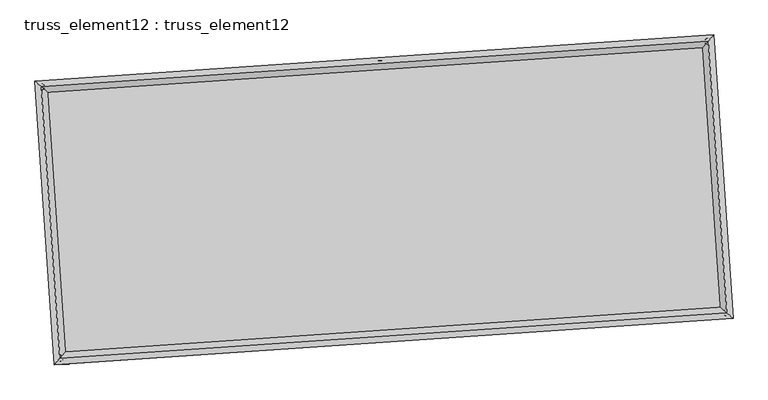
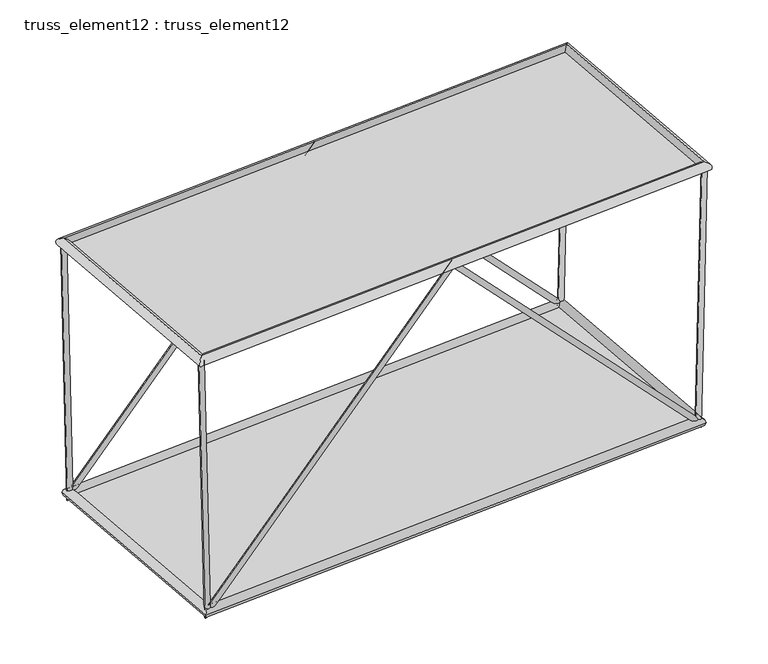
"""IFC4 building model written with IfcOpenShell, lengths in millimetres: plate geometry, truss_element12 : truss_element12."""

import ifcopenshell
import ifcopenshell.guid

model = None  # the IFC model being written
_history = None  # IfcOwnerHistory: only IFC2X3 demands one
_inside = {}  # id of a spatial element -> (the spatial element, [elements in it])
_under = {}  # id of a project, library or spatial element -> (it, [spatial elements below it])
_declared = {}  # id of a project -> (the project, [libraries it declares])
_typed = {}  # id of a type object -> (the type object, [elements of that type])
_made_of = {}  # id of a material, layer set ... -> (it, [elements and type objects made of it])


def new_model(schema):
    """Start an empty IFC model of exactly this schema.

    Asked for "IFC4X3", IfcOpenShell would pick the latest addendum, in which some entities
    have other attributes; the version numbers below select the first issue.
    IFC2X3 requires an IfcOwnerHistory on every rooted entity: one is made here for all.
    """
    global model, _history
    if schema == "IFC4X3":
        model = ifcopenshell.file(schema_version=(4, 3, 0, 0))
    else:
        model = ifcopenshell.file(schema=schema)
    _inside.clear()
    _under.clear()
    _declared.clear()
    _typed.clear()
    _made_of.clear()
    _history = None
    if model.schema == "IFC2X3":
        org = make("IfcOrganization", Name="unknown")
        user = make(
            "IfcPersonAndOrganization",
            ThePerson=make("IfcPerson", FamilyName="unknown"),
            TheOrganization=org,
        )
        app = make(
            "IfcApplication",
            ApplicationDeveloper=org,
            Version="unknown",
            ApplicationFullName="unknown",
            ApplicationIdentifier="unknown",
        )
        _history = make(
            "IfcOwnerHistory",
            OwningUser=user,
            OwningApplication=app,
            ChangeAction="ADDED",
            CreationDate=0,
        )
    return model


def make(cls, **values):
    """One entity of the class cls with the attributes given. An attribute that is None is left unset."""
    return model.create_entity(
        cls, **{name: value for name, value in values.items() if value is not None}
    )


def rooted(cls, **values):
    """An entity with a GlobalId (a new one), such as an element, a storey or a relation."""
    return make(cls, GlobalId=ifcopenshell.guid.new(), OwnerHistory=_history, **values)


def si_unit(unit_type, name, prefix=None):
    """IfcSIUnit, for example si_unit("LENGTHUNIT", "METRE", prefix="MILLI")."""
    return make("IfcSIUnit", UnitType=unit_type, Prefix=prefix, Name=name)


def assignment(units):
    """IfcUnitAssignment: the units of a project."""
    return None if units is None else make("IfcUnitAssignment", Units=units)


def point(xyz):
    """IfcCartesianPoint."""
    return None if xyz is None else make("IfcCartesianPoint", Coordinates=xyz)


def direction(xyz):
    """IfcDirection."""
    return None if xyz is None else make("IfcDirection", DirectionRatios=xyz)


def frame(location, z_axis=None, x_axis=None):
    """IfcAxis2Placement3D, a coordinate frame: its origin and axes. An axis left out is left unset."""
    return make(
        "IfcAxis2Placement3D",
        Location=point(location),
        Axis=direction(z_axis),
        RefDirection=direction(x_axis),
    )


def origin():
    """The frame at (0, 0, 0) with its axes left unset."""
    return frame((0.0, 0.0, 0.0))


def origin_with_axes():
    """The frame at (0, 0, 0) with the z axis (0, 0, 1) and the x axis (1, 0, 0) written out."""
    return frame((0.0, 0.0, 0.0), z_axis=(0.0, 0.0, 1.0), x_axis=(1.0, 0.0, 0.0))


def place(relative_to, where):
    """IfcLocalPlacement: puts the frame where relative to a parent placement (None: the world)."""
    return make(
        "IfcLocalPlacement", PlacementRelTo=relative_to, RelativePlacement=where
    )


def context(
    kind, dimensions, precision=None, world=None, true_north=None, identifier=None
):
    """IfcGeometricRepresentationContext, for example the 3D "Model" context."""
    return make(
        "IfcGeometricRepresentationContext",
        ContextIdentifier=identifier,
        ContextType=kind,
        CoordinateSpaceDimension=dimensions,
        Precision=precision,
        WorldCoordinateSystem=world,
        TrueNorth=true_north,
    )


def project(units=None, contexts=None):
    """IfcProject with its units and contexts."""
    return rooted(
        "IfcProject",
        Name="project",
        RepresentationContexts=contexts,
        UnitsInContext=assignment(units),
    )


def spatial(cls, under=None, at=None, **own):
    """A site, building, storey or space (cls), placed at a placement, below another one or the project."""
    s = rooted(cls, ObjectPlacement=at, **own)
    if under is not None:
        _under.setdefault(under.id(), (under, []))[1].append(s)
    return s


def polyline(points):
    """IfcPolyline through the points."""
    return make("IfcPolyline", Points=[point(p) for p in points])


def circle_curve(where, radius):
    """IfcCircle in the frame where."""
    return make("IfcCircle", Position=where, Radius=radius)


def ellipse_curve(where, semi_axis1, semi_axis2):
    """IfcEllipse in the frame where."""
    return make(
        "IfcEllipse", Position=where, SemiAxis1=semi_axis1, SemiAxis2=semi_axis2
    )


def outline(outer, holes=None, kind="AREA"):
    """IfcArbitraryClosedProfileDef: a profile drawn as a closed curve; with holes, ...WithVoids."""
    if holes is None:
        return make("IfcArbitraryClosedProfileDef", ProfileType=kind, OuterCurve=outer)
    return make(
        "IfcArbitraryProfileDefWithVoids",
        ProfileType=kind,
        OuterCurve=outer,
        InnerCurves=holes,
    )


def extrude(swept, where, along, depth):
    """IfcExtrudedAreaSolid: the profile swept, set in the frame where, extruded along a direction by depth."""
    return make(
        "IfcExtrudedAreaSolid",
        SweptArea=swept,
        Position=where,
        ExtrudedDirection=direction(along),
        Depth=depth,
    )


def shape(context_of_items, identifier, shape_type, items):
    """IfcShapeRepresentation: the items that make up one representation, for example the "Body"."""
    return make(
        "IfcShapeRepresentation",
        ContextOfItems=context_of_items,
        RepresentationIdentifier=identifier,
        RepresentationType=shape_type,
        Items=items,
    )


def source(mapping_origin, context_of_items, identifier, shape_type, items):
    """IfcRepresentationMap: a shape defined once, which mapped items show again and again."""
    return make(
        "IfcRepresentationMap",
        MappingOrigin=mapping_origin,
        MappedRepresentation=shape(context_of_items, identifier, shape_type, items),
    )


def transform(
    local_origin,
    x_axis=None,
    y_axis=None,
    z_axis=None,
    scale=None,
    scale2=None,
    scale3=None,
    uniform=True,
):
    """IfcCartesianTransformationOperator3D, or its non-uniform kind. x_axis, y_axis, z_axis: its Axis1, 2, 3."""
    if uniform:
        return make(
            "IfcCartesianTransformationOperator3D",
            Axis1=direction(x_axis),
            Axis2=direction(y_axis),
            LocalOrigin=point(local_origin),
            Scale=scale,
            Axis3=direction(z_axis),
        )
    return make(
        "IfcCartesianTransformationOperator3DnonUniform",
        Axis1=direction(x_axis),
        Axis2=direction(y_axis),
        LocalOrigin=point(local_origin),
        Scale=scale,
        Axis3=direction(z_axis),
        Scale2=scale2,
        Scale3=scale3,
    )


def mapped(mapping_source, mapping_target):
    """IfcMappedItem: shows the shape of a source again, moved by a transform."""
    return make(
        "IfcMappedItem", MappingSource=mapping_source, MappingTarget=mapping_target
    )


def made_of(thing, what):
    """Note that an element or type object is made of a material, layer set ...; save() writes the relation."""
    if what is not None:
        _made_of.setdefault(what.id(), (what, []))[1].append(thing)
    return thing


def element(
    cls,
    number,
    at=None,
    inside=None,
    cuts=None,
    type_object=None,
    material=None,
    context=None,
    identifier="Body",
    shape_type=None,
    held_by="IfcProductDefinitionShape",
    body=None,
    shapes=None,
    **own,
):
    """One element of the class cls, such as IfcWall. Its Tag is "e" and its number.

    at: its placement. inside: the storey or other place that contains it. cuts: it is an
    opening in that element (IfcRelVoidsElement). A single representation is given by context,
    identifier, shape_type and body (its items); several are given by shapes. held_by: the class
    of the entity that holds the representations. save() writes the other relations.
    """
    e = rooted(cls, Tag="e%d" % number, ObjectPlacement=at, **own)
    if body is not None:
        shapes = [shape(context, identifier, shape_type, body)]
    if shapes is not None:
        e.Representation = make(held_by, Representations=shapes)
    if inside is not None:
        _inside.setdefault(inside.id(), (inside, []))[1].append(e)
    if cuts is not None:
        rooted(
            "IfcRelVoidsElement", RelatingBuildingElement=cuts, RelatedOpeningElement=e
        )
    if type_object is not None:
        _typed.setdefault(type_object.id(), (type_object, []))[1].append(e)
    return made_of(e, material)


def aggregate(whole, parts):
    """IfcRelAggregates: a whole, such as a stair, and the parts it consists of."""
    return rooted("IfcRelAggregates", RelatingObject=whole, RelatedObjects=parts)


def save(model, path):
    """Write the relations noted so far, then the file.

    IfcRelAggregates (storeys below a building ...), IfcRelContainedInSpatialStructure (elements
    in a storey), IfcRelDefinesByType, IfcRelAssociatesMaterial and IfcRelDeclares: one each for
    every whole, place, type object, material and project.
    """
    for whole, parts in _under.values():
        aggregate(whole, parts)
    for where, things in _inside.values():
        rooted(
            "IfcRelContainedInSpatialStructure",
            RelatedElements=things,
            RelatingStructure=where,
        )
    for kind, things in _typed.values():
        rooted("IfcRelDefinesByType", RelatedObjects=things, RelatingType=kind)
    for what, things in _made_of.values():
        rooted("IfcRelAssociatesMaterial", RelatedObjects=things, RelatingMaterial=what)
    for by, libraries in _declared.values():
        rooted("IfcRelDeclares", RelatingContext=by, RelatedDefinitions=libraries)
    model.write(path)


def plane_surface(at):
    """IfcPlane: the flat surface through the origin of the frame at, square to its z axis."""
    return make("IfcPlane", Position=at)


def cylinder_surface(at, radius):
    """IfcCylindricalSurface: all points at the distance radius from the z axis of the frame at."""
    return make("IfcCylindricalSurface", Position=at, Radius=radius)


def advanced_brep(points, edges, surfaces, faces):
    """IfcAdvancedBrep: a solid bounded by faces that lie on surfaces and meet in shared edges.

    An edge is (start, end): straight between two places in points (the first is 0);
    or (start, end, curve); or (start, end, curve, False) where it runs against its curve.
    A face is (place in surfaces, loops), or (place, loops, False) where it looks against
    its surface's normal. A loop lists edges by number (the first is 1), with a minus sign
    where the edge is run from its end to its start. The first loop is the outer one.
    """
    corners = [point(p) for p in points]
    vertices = [make("IfcVertexPoint", VertexGeometry=c) for c in corners]
    made = []
    for start, end, *more in edges:
        made.append(
            make(
                "IfcEdgeCurve",
                EdgeStart=vertices[start],
                EdgeEnd=vertices[end],
                EdgeGeometry=more[0] if more else make("IfcPolyline", Points=[corners[start], corners[end]]),
                SameSense=more[1] if len(more) > 1 else True,
            )
        )
    hull = []
    for where, loops, *sense in faces:
        bounds = []
        for j, loop in enumerate(loops):
            ring = [make("IfcOrientedEdge", EdgeElement=made[abs(k) - 1], Orientation=k > 0) for k in loop]
            bounds.append(
                make(
                    "IfcFaceOuterBound" if j == 0 else "IfcFaceBound",
                    Bound=make("IfcEdgeLoop", EdgeList=ring),
                    Orientation=True,
                )
            )
        hull.append(make("IfcAdvancedFace", Bounds=bounds, FaceSurface=surfaces[where], SameSense=sense[0] if sense else True))
    return make("IfcAdvancedBrep", Outer=make("IfcClosedShell", CfsFaces=hull))


def truss_element12_truss_element12_a892e973(model_context):
    return source(origin(), model_context, "Body", "SolidModel", [
        advanced_brep(
        [(-3781.9001647, 2268.2490038, 4999.7954617), (-3880.9761734, 2254.8896434, 4997.4562298), (-3667.764278, 2276.0314961, 121.2292813), (-3761.2226048, 2263.055184, -121.2292813), (1063.7843207, 2598.6578087, 5070.7379408), (1064.2315522, 2592.0845597, 4926.5107211), (5795.2062001, 2921.2754808, 121.228402), (5889.5547769, 2921.1050077, -121.228402), (5909.4678674, 2929.0665496, 4999.7937205), (6009.4402165, 2929.2795401, 4997.4519118)],
        [
            (0, 1, circle_curve(frame((-3831.4381691, 2261.5693236, 4998.6258457), z_axis=(-0.02338894552682542, -0.0015948032857686179, 0.9997251691488132), x_axis=(-0.13359419431199426, 0.9910349164502389, -0.0015445460813113196)), 50.0)),
            (1, 0, circle_curve(frame((-3831.4381691, 2261.5693236, 4998.6258457), z_axis=(-0.02338894552682542, -0.0015948032857686179, 0.9997251691488132), x_axis=(-0.13359419431199426, 0.9910349164502389, -0.0015445460813113196)), 50.0)),
            (0, 2),
            (2, 3, ellipse_curve(frame((-3714.4934414, 2269.54334, 0.0), z_axis=(-0.9300590534640556, -0.06341719137026212, 0.36189558840672914), x_axis=(0.3610572196661413, 0.024619119302049103, 0.9322186348125354)), 130.3269965, 50.0)),
            (3, 1),
            (3, 2, ellipse_curve(frame((-3714.4934414, 2269.54334, 0.0), z_axis=(-0.9300590534640556, -0.06341719137026212, 0.36189558840672914), x_axis=(0.3610572196661413, 0.024619119302049103, 0.9322186348125354)), 130.3269965, 50.0)),
            (2, 4),
            (4, 5, ellipse_curve(frame((1064.0079364, 2595.3711842, 4998.6243309), z_axis=(-0.997683396052257, -0.06802823822715924, 6.733807032577008e-06), x_axis=(-6.718207468772972e-06, -4.580890289962869e-07, -0.9999999999773278)), 72.2706352, 50.0)),
            (5, 3),
            (5, 4, ellipse_curve(frame((1064.0079364, 2595.3711842, 4998.6243309), z_axis=(-0.997683396052257, -0.06802823822715924, 6.733807032577008e-06), x_axis=(-6.718207468772972e-06, -4.580890289962869e-07, -0.9999999999773278)), 72.2706352, 50.0)),
            (4, 6),
            (6, 7, ellipse_curve(frame((5842.3804885, 2921.1902443, 0.0), z_axis=(-0.9300661480063922, -0.06341767512013534, -0.3618772703761719), x_axis=(-0.3610389440712053, -0.024617873158702383, 0.9322257458282791)), 130.3250571, 50.0)),
            (7, 5),
            (7, 6, ellipse_curve(frame((5842.3804885, 2921.1902443, 0.0), z_axis=(-0.9300661480063922, -0.06341767512013534, -0.3618772703761719), x_axis=(-0.3610389440712053, -0.024617873158702383, 0.9322257458282791)), 130.3250571, 50.0)),
            (8, 9, circle_curve(frame((5959.4540419, 2929.1730448, 4998.6228161), z_axis=(0.02341471068854339, 0.0015965601142037436, 0.9997245632268789), x_axis=(-0.0021667064549673746, 0.9999964572445558, -0.0015462475466263355)), 50.0)),
            (9, 8, circle_curve(frame((5959.4540419, 2929.1730448, 4998.6228161), z_axis=(0.02341471068854339, 0.0015965601142037436, 0.9997245632268789), x_axis=(-0.0021667064549673746, 0.9999964572445558, -0.0015462475466263355)), 50.0)),
            (6, 8),
            (9, 7),
        ],
        [
            plane_surface(frame((-3831.4381691, 2311.56926, 4998.7056077), z_axis=(-0.023388945526825605, -0.0015948032857737312, 0.9997251691488132), x_axis=(0.9997264411963621, -3.731097392201122e-05, 0.023388915766833666))),
            cylinder_surface(frame((-3831.4381691, 2261.5693236, 4998.6258457), z_axis=(-0.02338894552682542, -0.0015948032857686179, 0.9997251691488132), x_axis=(-0.13359419431199426, 0.9910349164502389, -0.0015445460813113196)), 50.0),
            cylinder_surface(frame((-3714.4934414, 2269.54334, 0.0), z_axis=(-0.6902460485200175, -0.04706525417770467, -0.7220424186650602), x_axis=(-0.0204192616913266, 0.9987518848874466, -0.04558208184971222)), 50.0),
            cylinder_surface(frame((1064.0079364, 2595.3711842, 4998.6243309), z_axis=(-0.6902363467958805, -0.04706459265401546, 0.7220517361520492), x_axis=(-0.11534221170273892, 0.9922794497620825, -0.045581441172688954)), 50.0),
            plane_surface(frame((5959.4540419, 2879.1731086, 4998.702666), z_axis=(0.02341471068854475, 0.0015965601141989436, 0.999724563226879), x_axis=(0.9997258380793066, -3.739324497509243e-05, -0.023414680830057922))),
            cylinder_surface(frame((5842.3804885, 2921.1902443, 0.0), z_axis=(-0.02341471068854339, -0.0015965601142037436, -0.9997245632268789), x_axis=(-0.0021667064549673746, 0.9999964572445558, -0.0015462475466263355)), 50.0),
        ],
        [
            (0, [[1, 2]]),
            (1, [[-1, 3, 4, 5]]),
            (1, [[-2, -5, 6, -3]]),
            (2, [[-4, 7, 8, 9]]),
            (2, [[-6, -9, 10, -7]]),
            (3, [[-8, 11, 12, 13]]),
            (3, [[-10, -13, 14, -11]]),
            (4, [[15, 16]]),
            (5, [[-12, 17, -16, 18]]),
            (5, [[-14, -18, -15, -17]]),
        ],
    ),
        advanced_brep(
        [(-3509.7872118, -1722.4845805, 4999.7954617), (-3608.8632204, -1735.8439409, 4997.4562298), (-3395.6513251, -1714.7020882, 121.2292813), (-3489.1096519, -1727.6784003, -121.2292813), (1335.8972737, -1392.0757756, 5070.7379408), (1336.3445051, -1398.6490246, 4926.5107211), (6067.319153, -1069.4581035, 121.228402), (6161.6677299, -1069.6285766, -121.228402), (6181.5808204, -1061.6670347, 4999.7937205), (6281.5531694, -1061.4540442, 4997.4519118)],
        [
            (0, 1, circle_curve(frame((-3559.3252161, -1729.1642607, 4998.6258457), z_axis=(-0.023388945526825546, -0.0015948032857685606, 0.9997251691488132), x_axis=(-0.1335941943119938, 0.991034916450239, -0.0015445460813113816)), 50.0)),
            (1, 0, circle_curve(frame((-3559.3252161, -1729.1642607, 4998.6258457), z_axis=(-0.023388945526825546, -0.0015948032857685606, 0.9997251691488132), x_axis=(-0.1335941943119938, 0.991034916450239, -0.0015445460813113816)), 50.0)),
            (0, 2),
            (2, 3, ellipse_curve(frame((-3442.3804885, -1721.1902443, 0.0), z_axis=(-0.9300590534640557, -0.06341719137026187, 0.36189558840672914), x_axis=(0.36105721966614135, 0.024619119302049068, 0.9322186348125354)), 130.3269965, 50.0)),
            (3, 1),
            (3, 2, ellipse_curve(frame((-3442.3804885, -1721.1902443, 0.0), z_axis=(-0.9300590534640557, -0.06341719137026187, 0.36189558840672914), x_axis=(0.36105721966614135, 0.024619119302049068, 0.9322186348125354)), 130.3269965, 50.0)),
            (2, 4),
            (4, 5, ellipse_curve(frame((1336.1208894, -1395.3624001, 4998.6243309), z_axis=(-0.997683396052257, -0.06802823822715906, 6.733807032737481e-06), x_axis=(-6.718207468926731e-06, -4.580890289866768e-07, -0.9999999999773278)), 72.2706352, 50.0)),
            (5, 3),
            (5, 4, ellipse_curve(frame((1336.1208894, -1395.3624001, 4998.6243309), z_axis=(-0.997683396052257, -0.06802823822715906, 6.733807032737481e-06), x_axis=(-6.718207468926731e-06, -4.580890289866768e-07, -0.9999999999773278)), 72.2706352, 50.0)),
            (4, 6),
            (6, 7, ellipse_curve(frame((6114.4934414, -1069.54334, 0.0), z_axis=(-0.9300661480063922, -0.06341767512013499, -0.36187727037617134), x_axis=(-0.36103894407120507, -0.024617873158702393, 0.9322257458282792)), 130.3250571, 50.0)),
            (7, 5),
            (7, 6, ellipse_curve(frame((6114.4934414, -1069.54334, 0.0), z_axis=(-0.9300661480063922, -0.06341767512013499, -0.36187727037617134), x_axis=(-0.36103894407120507, -0.024617873158702393, 0.9322257458282792)), 130.3250571, 50.0)),
            (8, 9, circle_curve(frame((6231.5669949, -1061.5605395, 4998.6228161), z_axis=(0.023414710688543654, 0.0015965601142036118, 0.9997245632268787), x_axis=(-0.002166706454967089, 0.9999964572445559, -0.0015462475466262102)), 50.0)),
            (9, 8, circle_curve(frame((6231.5669949, -1061.5605395, 4998.6228161), z_axis=(0.023414710688543654, 0.0015965601142036118, 0.9997245632268787), x_axis=(-0.002166706454967089, 0.9999964572445559, -0.0015462475466262102)), 50.0)),
            (6, 8),
            (9, 7),
        ],
        [
            plane_surface(frame((-3559.3252161, -1679.1643243, 4998.7056077), z_axis=(-0.023388945526825605, -0.0015948032857737268, 0.9997251691488132), x_axis=(0.9997264411963621, -3.731097392201122e-05, 0.023388915766833666))),
            cylinder_surface(frame((-3559.3252161, -1729.1642607, 4998.6258457), z_axis=(-0.023388945526825546, -0.0015948032857685606, 0.9997251691488132), x_axis=(-0.1335941943119938, 0.991034916450239, -0.0015445460813113816)), 50.0),
            cylinder_surface(frame((-3442.3804885, -1721.1902443, 0.0), z_axis=(-0.6902460485200175, -0.04706525417770453, -0.7220424186650602), x_axis=(-0.020419261691326598, 0.9987518848874467, -0.04558208184971204)), 50.0),
            cylinder_surface(frame((1336.1208894, -1395.3624001, 4998.6243309), z_axis=(-0.6902363467958806, -0.047064592654015365, 0.7220517361520495), x_axis=(-0.11534221170273865, 0.9922794497620827, -0.0455814411726888)), 50.0),
            plane_surface(frame((6231.5669949, -1111.5604757, 4998.702666), z_axis=(0.02341471068854475, 0.0015965601141989436, 0.999724563226879), x_axis=(0.9997258380793066, -3.739324497464834e-05, -0.023414680830057922))),
            cylinder_surface(frame((6114.4934414, -1069.54334, 0.0), z_axis=(-0.023414710688543658, -0.0015965601142036122, -0.999724563226879), x_axis=(-0.002166706454967089, 0.9999964572445559, -0.0015462475466262102)), 50.0),
        ],
        [
            (0, [[1, 2]]),
            (1, [[-1, 3, 4, 5]]),
            (1, [[-2, -5, 6, -3]]),
            (2, [[-4, 7, 8, 9]]),
            (2, [[-6, -9, 10, -7]]),
            (3, [[-8, 11, 12, 13]]),
            (3, [[-10, -13, 14, -11]]),
            (4, [[15, 16]]),
            (5, [[-12, 17, -16, 18]]),
            (5, [[-14, -18, -15, -17]]),
        ],
    ),
        advanced_brep(
        [(-3559.3260024, -1729.1651321, 4908.6258457), (-3559.3244299, -1729.1633893, 5088.6258457), (-3831.4372718, 2261.568567, 5088.6258457), (-3831.4390663, 2261.5700802, 4908.6258457), (5959.4533112, 2929.1721772, 5088.6228161), (5959.4547727, 2929.1739124, 4908.6228161), (6231.5661531, -1061.5597791, 5088.6228161), (6231.5678367, -1061.5612999, 4908.6228161)],
        [
            (0, 1, ellipse_curve(frame((-3559.3252161, -1729.1642607, 4998.6258457), z_axis=(-0.7535719234054201, 0.6573654662780878, 2.1829417809630158e-07), x_axis=(-0.6573654662780518, -0.7535719234054518, 2.182941780963455e-07)), 127.2792206, 90.0)),
            (1, 2),
            (2, 3, ellipse_curve(frame((-3831.4381691, 2261.5693236, 4998.6258457), z_axis=(-0.6573654662780518, -0.7535719234054514, 2.1829417809638662e-07), x_axis=(0.7535719234054199, -0.6573654662780882, -2.1829417809634269e-07)), 127.2792206, 90.0)),
            (3, 0),
            (1, 0, ellipse_curve(frame((-3559.3252161, -1729.1642607, 4998.6258457), z_axis=(-0.7535719234054201, 0.6573654662780878, 2.1829417809630158e-07), x_axis=(-0.6573654662780518, -0.7535719234054518, 2.182941780963455e-07)), 127.2792206, 90.0)),
            (3, 2, ellipse_curve(frame((-3831.4381691, 2261.5693236, 4998.6258457), z_axis=(-0.6573654662780518, -0.7535719234054514, 2.1829417809638662e-07), x_axis=(0.7535719234054199, -0.6573654662780882, -2.1829417809634269e-07)), 127.2792206, 90.0)),
            (2, 4),
            (4, 5, ellipse_curve(frame((5959.4540419, 2929.1730448, 4998.6228161), z_axis=(-0.7535719234054205, 0.6573654662780875, 2.1829417809638398e-07), x_axis=(-0.6573654662780517, -0.7535719234054518, 2.182941780963455e-07)), 127.2792206, 90.0)),
            (5, 3),
            (5, 4, ellipse_curve(frame((5959.4540419, 2929.1730448, 4998.6228161), z_axis=(-0.7535719234054205, 0.6573654662780875, 2.1829417809638398e-07), x_axis=(-0.6573654662780517, -0.7535719234054518, 2.182941780963455e-07)), 127.2792206, 90.0)),
            (4, 6),
            (6, 7, ellipse_curve(frame((6231.5669949, -1061.5605395, 4998.6228161), z_axis=(0.6573654662780518, 0.7535719234054516, -2.182941780963044e-07), x_axis=(-0.7535719234054203, 0.6573654662780877, 2.1829417809634276e-07)), 127.2792206, 90.0)),
            (7, 5),
            (7, 6, ellipse_curve(frame((6231.5669949, -1061.5605395, 4998.6228161), z_axis=(0.6573654662780518, 0.7535719234054516, -2.182941780963044e-07), x_axis=(-0.7535719234054203, 0.6573654662780877, 2.1829417809634276e-07)), 127.2792206, 90.0)),
            (6, 1),
            (0, 7),
        ],
        [
            cylinder_surface(frame((-3559.3252161, -1729.1642607, 4998.6258457), z_axis=(0.068028238228695, -0.997683396074877, 0.0), x_axis=(-0.9976833960310403, -0.06802823822570593, 9.37427355396154e-06)), 90.0),
            cylinder_surface(frame((-3831.4381691, 2261.5693236, 4998.6258457), z_axis=(-0.9976833960748295, -0.06802823822869196, 3.0871458725096684e-07), x_axis=(-0.06802823822310758, 0.9976833960340704, 9.065558966723289e-06)), 90.0),
            cylinder_surface(frame((5959.4540419, 2929.1730448, 4998.6228161), z_axis=(-0.06802823822869553, 0.9976833960748772, 0.0), x_axis=(0.9976833960366247, 0.06802823822608724, 8.75684437948504e-06)), 90.0),
            cylinder_surface(frame((6231.5669949, -1061.5605395, 4998.6228161), z_axis=(0.9976833960748296, 0.06802823822869167, -3.0871458725090866e-07), x_axis=(0.06802823822869167, -0.9976833960336897, 9.065558966723292e-06)), 90.0),
        ],
        [
            (0, [[1, 2, 3, 4]]),
            (0, [[5, -4, 6, -2]]),
            (1, [[-3, 7, 8, 9]]),
            (1, [[-6, -9, 10, -7]]),
            (2, [[-8, 11, 12, 13]]),
            (2, [[-10, -13, 14, -11]]),
            (3, [[-12, 15, -1, 16]]),
            (3, [[-14, -16, -5, -15]]),
        ],
    ),
        advanced_brep(
        [(-3358.7115243, -1625.2761972, 0.0), (-3526.0494527, -1817.1042913, 0.0), (-3810.4074885, 2353.2123043, 0.0), (-3618.5793943, 2185.8743758, 0.0), (5926.0494527, 3017.1042913, 0.0), (5758.7115243, 2825.2761972, 0.0), (6210.4074885, -1153.2123043, 0.0), (6018.5793943, -985.8743758, 0.0)],
        [
            (0, 1, ellipse_curve(frame((-3442.3804885, -1721.1902443, 0.0), z_axis=(-0.7535719234054582, 0.6573654662780805, 0.0), x_axis=(-0.6573654662780803, -0.7535719234054584, 0.0)), 127.2792206, 90.0)),
            (1, 2),
            (2, 3, ellipse_curve(frame((-3714.4934414, 2269.54334, 0.0), z_axis=(-0.6573654662780803, -0.7535719234054584, 0.0), x_axis=(0.7535719234054584, -0.6573654662780801, 0.0)), 127.2792206, 90.0)),
            (3, 0),
            (1, 0, ellipse_curve(frame((-3442.3804885, -1721.1902443, 0.0), z_axis=(-0.7535719234054582, 0.6573654662780805, 0.0), x_axis=(-0.6573654662780803, -0.7535719234054584, 0.0)), 127.2792206, 90.0)),
            (3, 2, ellipse_curve(frame((-3714.4934414, 2269.54334, 0.0), z_axis=(-0.6573654662780803, -0.7535719234054584, 0.0), x_axis=(0.7535719234054584, -0.6573654662780801, 0.0)), 127.2792206, 90.0)),
            (2, 4),
            (4, 5, ellipse_curve(frame((5842.3804885, 2921.1902443, 0.0), z_axis=(-0.7535719234054583, 0.6573654662780803, 0.0), x_axis=(-0.6573654662780803, -0.7535719234054583, 0.0)), 127.2792206, 90.0)),
            (5, 3),
            (5, 4, ellipse_curve(frame((5842.3804885, 2921.1902443, 0.0), z_axis=(-0.7535719234054583, 0.6573654662780803, 0.0), x_axis=(-0.6573654662780803, -0.7535719234054583, 0.0)), 127.2792206, 90.0)),
            (4, 6),
            (6, 7, ellipse_curve(frame((6114.4934414, -1069.54334, 0.0), z_axis=(0.6573654662780806, 0.7535719234054582, 0.0), x_axis=(-0.7535719234054582, 0.6573654662780806, 0.0)), 127.2792206, 90.0)),
            (7, 5),
            (7, 6, ellipse_curve(frame((6114.4934414, -1069.54334, 0.0), z_axis=(0.6573654662780806, 0.7535719234054582, 0.0), x_axis=(-0.7535719234054582, 0.6573654662780806, 0.0)), 127.2792206, 90.0)),
            (6, 1),
            (0, 7),
        ],
        [
            cylinder_surface(frame((-3442.3804885, -1721.1902443, 0.0), z_axis=(0.06802823822870183, -0.9976833960748765, 0.0), x_axis=(-0.9976833960748765, -0.06802823822870183, 0.0)), 90.0),
            cylinder_surface(frame((-3714.4934414, 2269.54334, 0.0), z_axis=(-0.9976833960748765, -0.068028238228702, 0.0), x_axis=(-0.068028238228702, 0.9976833960748765, 0.0)), 90.0),
            cylinder_surface(frame((5842.3804885, 2921.1902443, 0.0), z_axis=(-0.06802823822870174, 0.9976833960748765, 0.0), x_axis=(0.9976833960748765, 0.06802823822870174, 0.0)), 90.0),
            cylinder_surface(frame((6114.4934414, -1069.54334, 0.0), z_axis=(0.9976833960748768, 0.06802823822870133, 0.0), x_axis=(0.06802823822870133, -0.9976833960748768, 0.0)), 90.0),
        ],
        [
            (0, [[1, 2, 3, 4]]),
            (0, [[5, -4, 6, -2]]),
            (1, [[-3, 7, 8, 9]]),
            (1, [[-6, -9, 10, -7]]),
            (2, [[-8, 11, 12, 13]]),
            (2, [[-10, -13, 14, -11]]),
            (3, [[-12, 15, -1, 16]]),
            (3, [[-14, -16, -5, -15]]),
        ],
    ),
        extrude(outline(polyline([(-3442.3804885, -1721.1902443), (-3714.4934414, 2269.54334), (5842.3804885, 2921.1902443), (6114.4934414, -1069.54334), (-3442.3804885, -1721.1902443)])), origin_with_axes(), (0.0, 0.0, 1.0), 20.0),
        extrude(outline(polyline([(-2000.0000001, 4906.8132483), (2000.0, 4906.8132484), (2000.0, -4906.8132483), (-2000.0000001, -4906.8132484), (-2000.0000001, 4906.8132483)])), frame((1200.0644129, 600.0043921, 4998.6243309), z_axis=(3.0799941782636943e-07, 2.1001309486182012e-08, 0.9999999999999525), x_axis=(-0.06802823822870138, 0.9976833960748767, 0.0)), (0.0, 0.0, 1.0), 20.0),
    ])


if __name__ == "__main__":
    model = new_model("IFC4")
    model_context = context("Model", 3, world=origin())
    ifc_project = project(units=[si_unit("LENGTHUNIT", "METRE", prefix="MILLI")], contexts=[model_context])
    site = spatial("IfcSite", under=ifc_project)
    building = spatial("IfcBuilding", under=site)
    placement = place(None, origin())
    truss_element12_truss_element12_shape = truss_element12_truss_element12_a892e973(model_context)
    element("IfcPlate", 1, ObjectType="truss_element12 : truss_element12", at=placement, inside=building, context=model_context, shape_type="MappedRepresentation", body=[
        mapped(truss_element12_truss_element12_shape, transform((0.0, 0.0, 0.0), x_axis=(1.0, 0.0, 0.0), y_axis=(0.0, 1.0, 0.0), z_axis=(0.0, 0.0, 1.0))),
    ])
    save(model, "model.ifc")

# Revit data of these elements
# Type "truss_element12 : truss_element12"
#   steellbar1 = 90 mm
#   steelbar2 = 50 mm
#   offset1 = 5000 mm
#   M = Default Roof
# Element 1 (IfcPlate, "truss_element12 : truss_element12")
#   Materials on its faces: "Default Roof"
# Materials
#   "Default Roof": class "Miscellaneous", colour RGB 0 127 0, transparency 0, Comments = "Rendering appearance not upgraded Rendering appearance not upgraded ", Cost = 0
